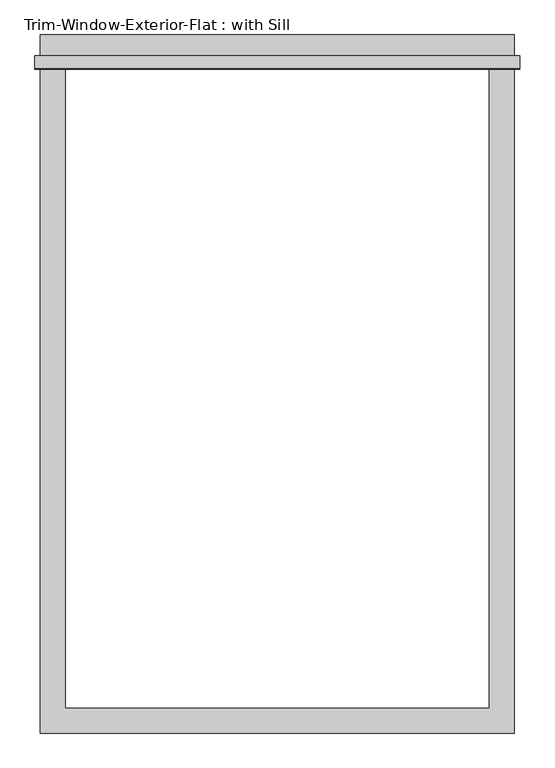
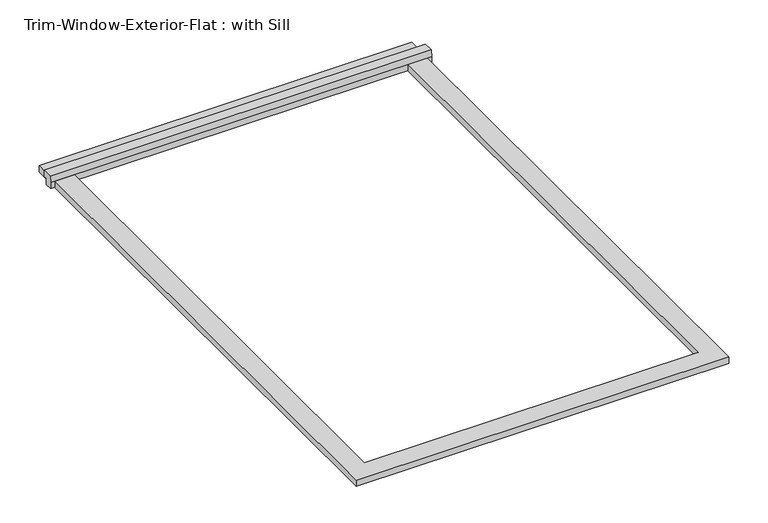
"""IFC4 building model written with IfcOpenShell, lengths in millimetres: proxy geometry, Trim-Window-Exterior-Flat : with Sill."""

import ifcopenshell
import ifcopenshell.guid

model = None  # the IFC model being written
_history = None  # IfcOwnerHistory: only IFC2X3 demands one
_inside = {}  # id of a spatial element -> (the spatial element, [elements in it])
_under = {}  # id of a project, library or spatial element -> (it, [spatial elements below it])
_declared = {}  # id of a project -> (the project, [libraries it declares])
_typed = {}  # id of a type object -> (the type object, [elements of that type])
_made_of = {}  # id of a material, layer set ... -> (it, [elements and type objects made of it])


def new_model(schema):
    """Start an empty IFC model of exactly this schema.

    Asked for "IFC4X3", IfcOpenShell would pick the latest addendum, in which some entities
    have other attributes; the version numbers below select the first issue.
    IFC2X3 requires an IfcOwnerHistory on every rooted entity: one is made here for all.
    """
    global model, _history
    if schema == "IFC4X3":
        model = ifcopenshell.file(schema_version=(4, 3, 0, 0))
    else:
        model = ifcopenshell.file(schema=schema)
    _inside.clear()
    _under.clear()
    _declared.clear()
    _typed.clear()
    _made_of.clear()
    _history = None
    if model.schema == "IFC2X3":
        org = make("IfcOrganization", Name="unknown")
        user = make(
            "IfcPersonAndOrganization",
            ThePerson=make("IfcPerson", FamilyName="unknown"),
            TheOrganization=org,
        )
        app = make(
            "IfcApplication",
            ApplicationDeveloper=org,
            Version="unknown",
            ApplicationFullName="unknown",
            ApplicationIdentifier="unknown",
        )
        _history = make(
            "IfcOwnerHistory",
            OwningUser=user,
            OwningApplication=app,
            ChangeAction="ADDED",
            CreationDate=0,
        )
    return model


def make(cls, **values):
    """One entity of the class cls with the attributes given. An attribute that is None is left unset."""
    return model.create_entity(
        cls, **{name: value for name, value in values.items() if value is not None}
    )


def rooted(cls, **values):
    """An entity with a GlobalId (a new one), such as an element, a storey or a relation."""
    return make(cls, GlobalId=ifcopenshell.guid.new(), OwnerHistory=_history, **values)


def si_unit(unit_type, name, prefix=None):
    """IfcSIUnit, for example si_unit("LENGTHUNIT", "METRE", prefix="MILLI")."""
    return make("IfcSIUnit", UnitType=unit_type, Prefix=prefix, Name=name)


def assignment(units):
    """IfcUnitAssignment: the units of a project."""
    return None if units is None else make("IfcUnitAssignment", Units=units)


def point(xyz):
    """IfcCartesianPoint."""
    return None if xyz is None else make("IfcCartesianPoint", Coordinates=xyz)


def direction(xyz):
    """IfcDirection."""
    return None if xyz is None else make("IfcDirection", DirectionRatios=xyz)


def frame(location, z_axis=None, x_axis=None):
    """IfcAxis2Placement3D, a coordinate frame: its origin and axes. An axis left out is left unset."""
    return make(
        "IfcAxis2Placement3D",
        Location=point(location),
        Axis=direction(z_axis),
        RefDirection=direction(x_axis),
    )


def origin():
    """The frame at (0, 0, 0) with its axes left unset."""
    return frame((0.0, 0.0, 0.0))


def origin_with_axes():
    """The frame at (0, 0, 0) with the z axis (0, 0, 1) and the x axis (1, 0, 0) written out."""
    return frame((0.0, 0.0, 0.0), z_axis=(0.0, 0.0, 1.0), x_axis=(1.0, 0.0, 0.0))


def place(relative_to, where):
    """IfcLocalPlacement: puts the frame where relative to a parent placement (None: the world)."""
    return make(
        "IfcLocalPlacement", PlacementRelTo=relative_to, RelativePlacement=where
    )


def context(
    kind, dimensions, precision=None, world=None, true_north=None, identifier=None
):
    """IfcGeometricRepresentationContext, for example the 3D "Model" context."""
    return make(
        "IfcGeometricRepresentationContext",
        ContextIdentifier=identifier,
        ContextType=kind,
        CoordinateSpaceDimension=dimensions,
        Precision=precision,
        WorldCoordinateSystem=world,
        TrueNorth=true_north,
    )


def project(units=None, contexts=None):
    """IfcProject with its units and contexts."""
    return rooted(
        "IfcProject",
        Name="project",
        RepresentationContexts=contexts,
        UnitsInContext=assignment(units),
    )


def spatial(cls, under=None, at=None, **own):
    """A site, building, storey or space (cls), placed at a placement, below another one or the project."""
    s = rooted(cls, ObjectPlacement=at, **own)
    if under is not None:
        _under.setdefault(under.id(), (under, []))[1].append(s)
    return s


def polyline(points):
    """IfcPolyline through the points."""
    return make("IfcPolyline", Points=[point(p) for p in points])


def outline(outer, holes=None, kind="AREA"):
    """IfcArbitraryClosedProfileDef: a profile drawn as a closed curve; with holes, ...WithVoids."""
    if holes is None:
        return make("IfcArbitraryClosedProfileDef", ProfileType=kind, OuterCurve=outer)
    return make(
        "IfcArbitraryProfileDefWithVoids",
        ProfileType=kind,
        OuterCurve=outer,
        InnerCurves=holes,
    )


def extrude(swept, where, along, depth):
    """IfcExtrudedAreaSolid: the profile swept, set in the frame where, extruded along a direction by depth."""
    return make(
        "IfcExtrudedAreaSolid",
        SweptArea=swept,
        Position=where,
        ExtrudedDirection=direction(along),
        Depth=depth,
    )


def shape(context_of_items, identifier, shape_type, items):
    """IfcShapeRepresentation: the items that make up one representation, for example the "Body"."""
    return make(
        "IfcShapeRepresentation",
        ContextOfItems=context_of_items,
        RepresentationIdentifier=identifier,
        RepresentationType=shape_type,
        Items=items,
    )


def source(mapping_origin, context_of_items, identifier, shape_type, items):
    """IfcRepresentationMap: a shape defined once, which mapped items show again and again."""
    return make(
        "IfcRepresentationMap",
        MappingOrigin=mapping_origin,
        MappedRepresentation=shape(context_of_items, identifier, shape_type, items),
    )


def transform(
    local_origin,
    x_axis=None,
    y_axis=None,
    z_axis=None,
    scale=None,
    scale2=None,
    scale3=None,
    uniform=True,
):
    """IfcCartesianTransformationOperator3D, or its non-uniform kind. x_axis, y_axis, z_axis: its Axis1, 2, 3."""
    if uniform:
        return make(
            "IfcCartesianTransformationOperator3D",
            Axis1=direction(x_axis),
            Axis2=direction(y_axis),
            LocalOrigin=point(local_origin),
            Scale=scale,
            Axis3=direction(z_axis),
        )
    return make(
        "IfcCartesianTransformationOperator3DnonUniform",
        Axis1=direction(x_axis),
        Axis2=direction(y_axis),
        LocalOrigin=point(local_origin),
        Scale=scale,
        Axis3=direction(z_axis),
        Scale2=scale2,
        Scale3=scale3,
    )


def mapped(mapping_source, mapping_target):
    """IfcMappedItem: shows the shape of a source again, moved by a transform."""
    return make(
        "IfcMappedItem", MappingSource=mapping_source, MappingTarget=mapping_target
    )


def made_of(thing, what):
    """Note that an element or type object is made of a material, layer set ...; save() writes the relation."""
    if what is not None:
        _made_of.setdefault(what.id(), (what, []))[1].append(thing)
    return thing


def element(
    cls,
    number,
    at=None,
    inside=None,
    cuts=None,
    type_object=None,
    material=None,
    context=None,
    identifier="Body",
    shape_type=None,
    held_by="IfcProductDefinitionShape",
    body=None,
    shapes=None,
    **own,
):
    """One element of the class cls, such as IfcWall. Its Tag is "e" and its number.

    at: its placement. inside: the storey or other place that contains it. cuts: it is an
    opening in that element (IfcRelVoidsElement). A single representation is given by context,
    identifier, shape_type and body (its items); several are given by shapes. held_by: the class
    of the entity that holds the representations. save() writes the other relations.
    """
    e = rooted(cls, Tag="e%d" % number, ObjectPlacement=at, **own)
    if body is not None:
        shapes = [shape(context, identifier, shape_type, body)]
    if shapes is not None:
        e.Representation = make(held_by, Representations=shapes)
    if inside is not None:
        _inside.setdefault(inside.id(), (inside, []))[1].append(e)
    if cuts is not None:
        rooted(
            "IfcRelVoidsElement", RelatingBuildingElement=cuts, RelatedOpeningElement=e
        )
    if type_object is not None:
        _typed.setdefault(type_object.id(), (type_object, []))[1].append(e)
    return made_of(e, material)


def aggregate(whole, parts):
    """IfcRelAggregates: a whole, such as a stair, and the parts it consists of."""
    return rooted("IfcRelAggregates", RelatingObject=whole, RelatedObjects=parts)


def save(model, path):
    """Write the relations noted so far, then the file.

    IfcRelAggregates (storeys below a building ...), IfcRelContainedInSpatialStructure (elements
    in a storey), IfcRelDefinesByType, IfcRelAssociatesMaterial and IfcRelDeclares: one each for
    every whole, place, type object, material and project.
    """
    for whole, parts in _under.values():
        aggregate(whole, parts)
    for where, things in _inside.values():
        rooted(
            "IfcRelContainedInSpatialStructure",
            RelatedElements=things,
            RelatingStructure=where,
        )
    for kind, things in _typed.values():
        rooted("IfcRelDefinesByType", RelatedObjects=things, RelatingType=kind)
    for what, things in _made_of.values():
        rooted("IfcRelAssociatesMaterial", RelatedObjects=things, RelatingMaterial=what)
    for by, libraries in _declared.values():
        rooted("IfcRelDeclares", RelatingContext=by, RelatedDefinitions=libraries)
    model.write(path)


def trim_window_exterior_flat_with_sill_c46fdb85(model_context):
    return source(origin(), model_context, "Body", "SweptSolid", [
        extrude(outline(polyline([(546.1, 1495.3823709), (-546.1, 1495.3823709), (-546.1, 1552.5323709), (546.1, 1552.5323709), (546.1, 1495.3823709)])), origin_with_axes(), (0.0, 0.0, 1.0), 19.05),
        extrude(outline(polyline([(1504.95, 38.1), (1504.95, 19.05), (1495.3823709, 19.05), (1495.3823709, 0.0), (1473.2, 0.0), (1473.2, 19.05), (1475.6580645, 38.1), (1504.95, 38.1)])), frame((-558.8, 0.0, 0.0), z_axis=(1.0, 0.0, 0.0), x_axis=(0.0, 1.0, 0.0)), (0.0, 0.0, 1.0), 1117.6),
        extrude(outline(polyline([(-546.1, -57.15), (-546.1, 1473.2), (-488.95, 1473.2), (-488.95, 0.0), (488.95, 0.0), (488.95, 1473.2), (546.1, 1473.2), (546.1, -57.15), (-546.1, -57.15)])), origin_with_axes(), (0.0, 0.0, 1.0), 19.05),
    ])


if __name__ == "__main__":
    model = new_model("IFC4")
    model_context = context("Model", 3, world=origin())
    ifc_project = project(units=[si_unit("LENGTHUNIT", "METRE", prefix="MILLI")], contexts=[model_context])
    site = spatial("IfcSite", under=ifc_project)
    building = spatial("IfcBuilding", under=site)
    placement = place(None, origin())
    trim_window_exterior_flat_with_sill_shape = trim_window_exterior_flat_with_sill_c46fdb85(model_context)
    element("IfcBuildingElementProxy", 1, Name="Trim-Window-Exterior-Flat : with Sill", ObjectType="Trim-Window-Exterior-Flat : with Sill", at=placement, inside=building, context=model_context, shape_type="MappedRepresentation", body=[
        mapped(trim_window_exterior_flat_with_sill_shape, transform((0.0, 0.0, 0.0), x_axis=(1.0, 0.0, 0.0), y_axis=(0.0, 1.0, 0.0), z_axis=(0.0, 0.0, 1.0))),
    ])
    save(model, "model.ifc")

# Revit data of these elements
# Type "Trim-Window-Exterior-Flat : with Sill"
#   Trim Width = 0' - 2 1/4"
#   Trim Thickness_Picture Frame = 0' - 1 1/4"
#   Trim Thickness_with Sill = 0' - 0 3/4"
#   Sill Thickness = 0' - 1 1/4"
#   Opening Width [instance default] = 2' - 0"
#   Opening Height [instance default] = 3' - 0"
#   Default Elevation = 4' - 0"
#   Sill = yes
#   Picture Frame = no
#   Trim Material [instance default] = none
# Element 1 (IfcBuildingElementProxy, "Trim-Window-Exterior-Flat : with Sill")
#   Opening Width = 3' - 2 1/2"
#   Opening Height = 4' - 10"
#   Trim Material = Clad - White
#   Materials on its faces: "Clad - White"
# Materials
#   "Clad - White": class "Wood", colour RGB 242 242 238, transparency 0, Cost = 0
